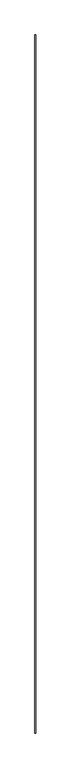
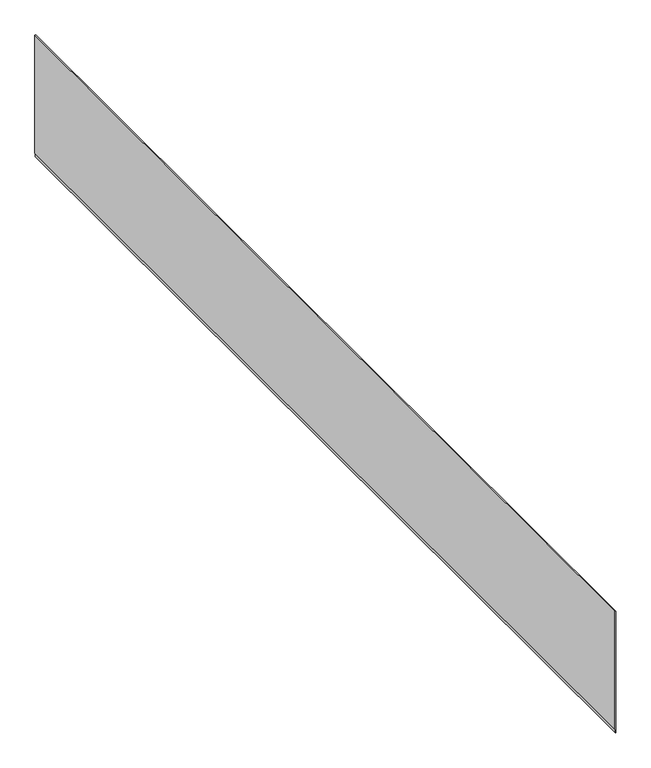
"""IFC4 building model written with IfcOpenShell, lengths in millimetres: proxy geometry, Generic Models 7:Generic Models 1:5:Generic Models 1:5 : Generic Models 7:Generic Models 1:337419:29 : Generic Models 7:Generic Models 1:5:Generic Models 1:5 : Generic Models 7:Generic Models 1:337419:311462."""

from ifc_helpers import new_model, si_unit, frame, origin, place, context, project, spatial, polyline, outline, extrude, source, transform, mapped, element, save


def generic_models_b64bfd4d(model_context):
    return source(origin(), model_context, "Body", "SweptSolid", [
        extrude(outline(polyline([(62.8710435, 0.0), (62.8710435, -9.7192949), (-2368.3852065, -9.7192949), (-2368.3852065, 9.3307051), (-9.1722618, 9.3307051), (1.9476395, 0.0), (62.8710435, 0.0)])), frame((579336.092429, -579019.7413841, 3786.7057425), z_axis=(1.043998221206266e-11, 1.0, 0.0), x_axis=(0.0, 0.0, -1.0)), (0.0, 0.0, 1.0), 18999.2000001),
    ])


if __name__ == "__main__":
    model = new_model("IFC4")
    model_context = context("Model", 3, world=origin())
    ifc_project = project(units=[si_unit("LENGTHUNIT", "METRE", prefix="MILLI")], contexts=[model_context])
    site = spatial("IfcSite", under=ifc_project)
    building = spatial("IfcBuilding", under=site)
    placement = place(None, origin())
    generic_models_shape = generic_models_b64bfd4d(model_context)
    element("IfcBuildingElementProxy", 1, Name="Generic Models 7:Generic Models 1:5:Generic Models 1:5 : Generic Models 7:Generic Models 1:337419:29 : Generic Models 7:Generic Models 1:5:Generic Models 1:5 : Generic Models 7:Generic Models 1:337419:311462", ObjectType="Generic Models 7:Generic Models 1:5:Generic Models 1:5 : Generic Models 7:Generic Models 1:337419:29 : Generic Models 7:Generic Models 1:5:Generic Models 1:5 : Generic Models 7:Generic Models 1:337419:311462", at=placement, inside=building, context=model_context, shape_type="MappedRepresentation", body=[
        mapped(generic_models_shape, transform((0.0, 0.0, 0.0), x_axis=(1.0, 0.0, 0.0), y_axis=(0.0, 1.0, 0.0), z_axis=(0.0, 0.0, 1.0))),
    ])
    save(model, "model.ifc")

# Revit data of these elements
# Type "Generic Models 7:Generic Models 1:5:Generic Models 1:5 : Generic Models 7:Generic Models 1:337419:29 : Generic Models 7:Generic Models 1:5:Generic Models 1:5 : Generic Models 7:Generic Models 1:337419:311462"
#   NameOverride = "Generic Models 7:Generic Models 1:5:Generic Models 1:5 : Generic Models 7:Generic Models 1:337419:311462"
#   ObjectTypeOverride = "Generic Models 1:5 : Generic Models 7:Generic Models 1:337419"
#   Reference = "Generic Models 1"
#   Tag = "311462"
# Element 1 (IfcBuildingElementProxy, "Generic Models 7:Generic Models 1:5:Generic Models 1:5 : Generic Models 7:Generic Models 1:337419:29 : Generic Models 7:Generic Models 1:5:Generic Models 1:5 : Generic Models 7:Generic Models 1:337419:311462")
#   Materials on its faces: "1\" MINERAL WOOL BOARD INSULATION"
# Materials
#   "1\" MINERAL WOOL BOARD INSULATION": class "Unassigned", colour RGB 205 188 106, transparency 0, Cost = 0
